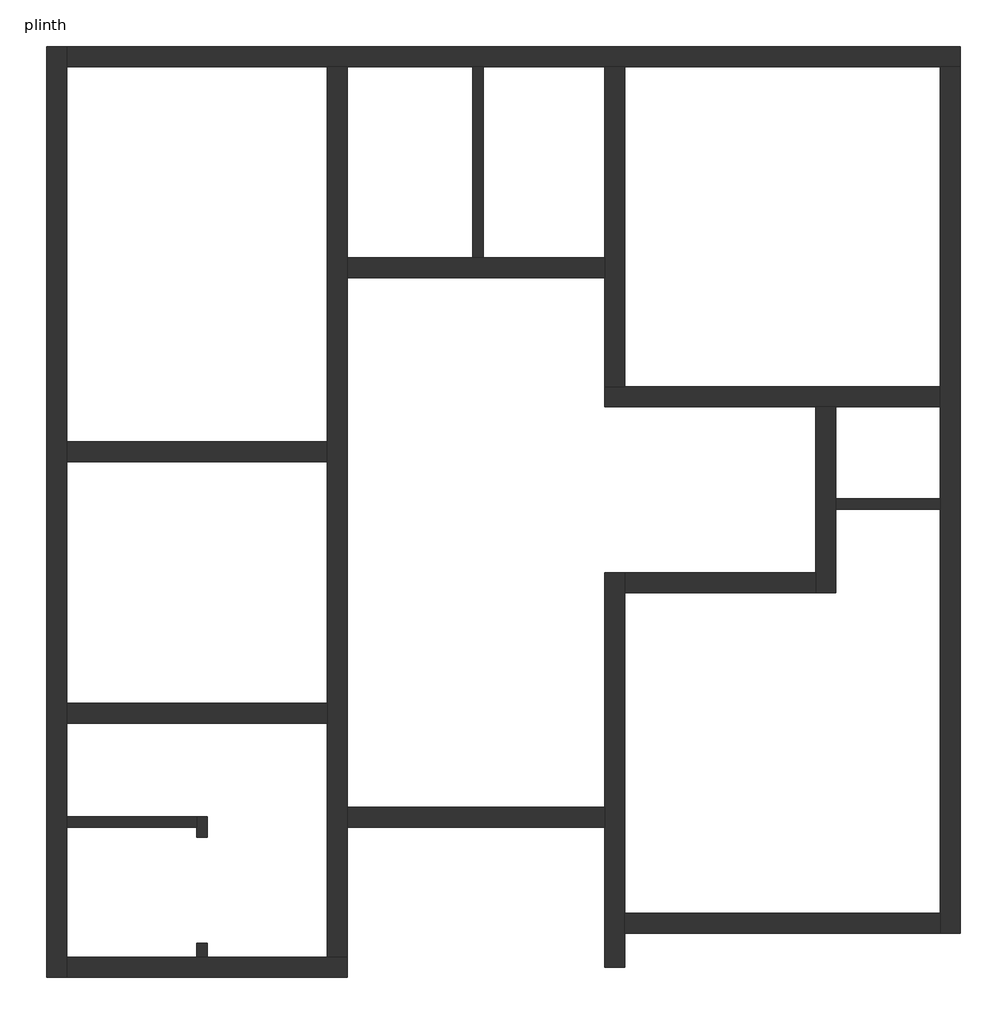
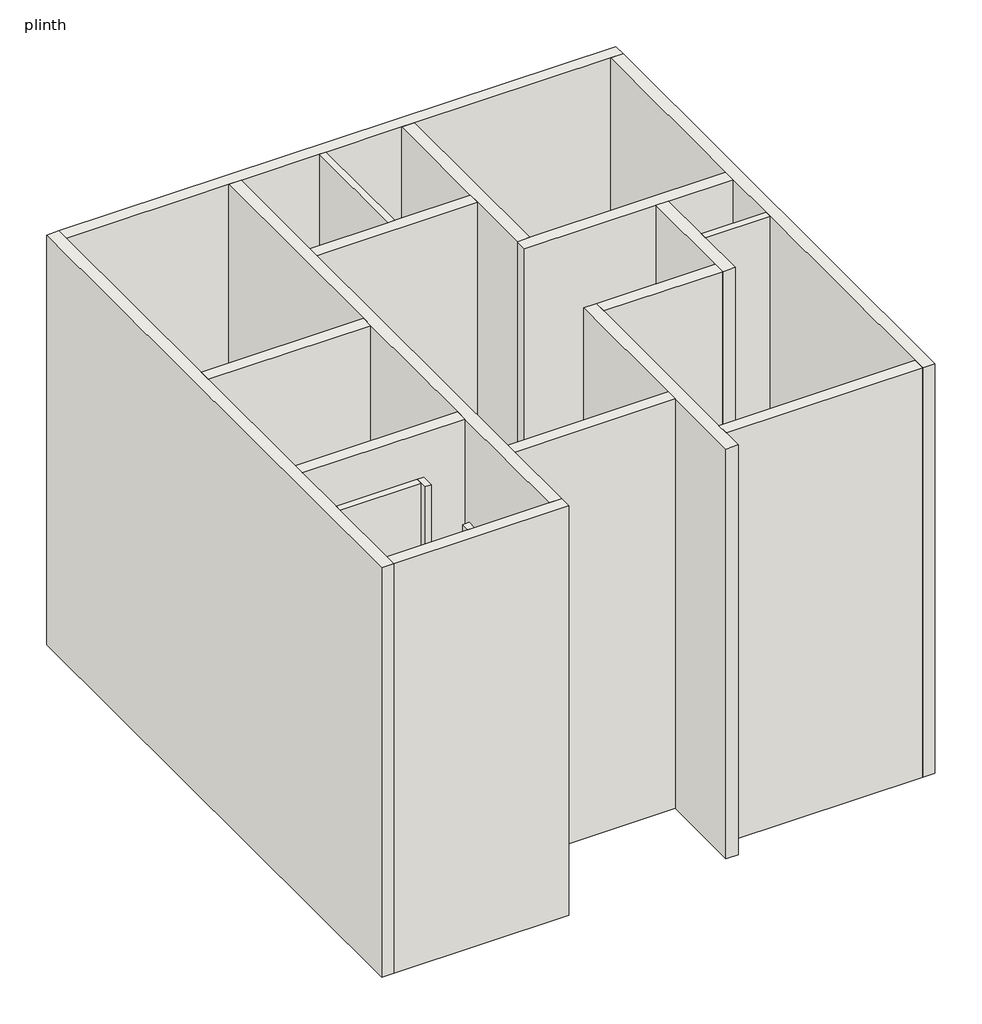
# One storey: 20 walls.
"""IFC4 building model written with IfcOpenShell, lengths in millimetres."""

from ifc_helpers import new_model, si_unit, frame, origin, place, context, project, spatial, polyline, outline, extrude, faceted_brep, element, save

model = new_model("IFC4")

# Units and contexts
model_context = context("Model", 3, world=origin())
ifc_project = project(units=[si_unit("LENGTHUNIT", "METRE", prefix="MILLI")], contexts=[model_context])

# Site, building, storey
site = spatial("IfcSite", under=ifc_project)
building = spatial("IfcBuilding", under=site)
storey = spatial("IfcBuildingStorey", under=building, Name="plinth", Elevation=450.0)

# Walls
placement = place(None, origin())
element("IfcWall", 1, ObjectType="11", at=placement, inside=storey, context=model_context, shape_type="SweptSolid", body=[
    extrude(outline(polyline([(-59261.991131, 24848.2615718), (-59261.991131, 22648.2615718), (-59381.991131, 22648.2615718), (-59381.991131, 24848.2615718), (-59261.991131, 24848.2615718)])), frame((0.0, 0.0, 450.0), z_axis=(0.0, 0.0, 1.0), x_axis=(1.0, 0.0, 0.0)), (0.0, 0.0, 1.0), 8000.0),
])
element("IfcWall", 2, ObjectType="111", at=placement, inside=storey, context=model_context, shape_type="SweptSolid", body=[
    extrude(outline(polyline([(-54001.991131, 19748.2615718), (-55201.991131, 19748.2615718), (-55201.991131, 19868.2615718), (-54001.991131, 19868.2615718), (-54001.991131, 19748.2615718)])), frame((0.0, 0.0, 450.0), z_axis=(0.0, 0.0, 1.0), x_axis=(1.0, 0.0, 0.0)), (0.0, 0.0, 1.0), 8000.0),
])
element("IfcWall", 3, ObjectType="111", at=placement, inside=storey, context=model_context, shape_type="Brep", body=[
    faceted_brep([(-62561.991131, 16208.2615718, 450.0), (-62561.991131, 16088.2615718, 450.0), (-62561.991131, 15973.2615718, 450.0), (-62561.991131, 15973.2615718, 8450.0), (-62561.991131, 16088.2615718, 8450.0), (-62561.991131, 16208.2615718, 8450.0), (-62441.991131, 16208.2615718, 450.0), (-62441.991131, 16208.2615718, 8450.0), (-62441.991131, 15973.2615718, 8450.0), (-62441.991131, 15973.2615718, 450.0)], [[[0, 1, 2, 3, 4, 5]], [[6, 7, 8, 9]], [[2, 1, 0, 6, 9]], [[3, 2, 9, 8]], [[5, 4, 3, 8, 7]], [[0, 5, 7, 6]]]),
])
element("IfcWall", 4, ObjectType="111", at=placement, inside=storey, context=model_context, shape_type="SweptSolid", body=[
    extrude(outline(polyline([(-62441.991131, 14753.2615718), (-62441.991131, 14588.2615718), (-62561.991131, 14588.2615718), (-62561.991131, 14753.2615718), (-62441.991131, 14753.2615718)])), frame((0.0, 0.0, 450.0), z_axis=(0.0, 0.0, 1.0), x_axis=(1.0, 0.0, 0.0)), (0.0, 0.0, 1.0), 8000.0),
])
element("IfcWall", 5, ObjectType="111", at=placement, inside=storey, context=model_context, shape_type="SweptSolid", body=[
    extrude(outline(polyline([(-64061.991131, 16208.2615718), (-62561.991131, 16208.2615718), (-62561.991131, 16088.2615718), (-64061.991131, 16088.2615718), (-64061.991131, 16208.2615718)])), frame((0.0, 0.0, 450.0), z_axis=(0.0, 0.0, 1.0), x_axis=(1.0, 0.0, 0.0)), (0.0, 0.0, 1.0), 8000.0),
])
element("IfcWall", 6, ObjectType="Generic - 200mm", at=placement, inside=storey, context=model_context, shape_type="Brep", body=[
    faceted_brep([(-64291.991131, 25078.2615718, 450.0), (-64291.991131, 14358.2615718, 450.0), (-64291.991131, 14358.2615718, 8450.0), (-64291.991131, 25078.2615718, 8450.0), (-64061.991131, 25078.2615718, 450.0), (-64061.991131, 25078.2615718, 8450.0), (-64061.991131, 24848.2615718, 8450.0), (-64061.991131, 20528.2615718, 8450.0), (-64061.991131, 20298.2615718, 8450.0), (-64061.991131, 17518.2615718, 8450.0), (-64061.991131, 17288.2615718, 8450.0), (-64061.991131, 16208.2615718, 8450.0), (-64061.991131, 16088.2615718, 8450.0), (-64061.991131, 14588.2615718, 8450.0), (-64061.991131, 14358.2615718, 8450.0), (-64061.991131, 14358.2615718, 450.0), (-64061.991131, 14588.2615718, 450.0), (-64061.991131, 16088.2615718, 450.0), (-64061.991131, 16208.2615718, 450.0), (-64061.991131, 17288.2615718, 450.0), (-64061.991131, 17518.2615718, 450.0), (-64061.991131, 20298.2615718, 450.0), (-64061.991131, 20528.2615718, 450.0), (-64061.991131, 24848.2615718, 450.0)], [[[0, 1, 2, 3]], [[4, 5, 6, 7, 8, 9, 10, 11, 12, 13, 14, 15, 16, 17, 18, 19, 20, 21, 22, 23]], [[1, 0, 4, 23, 22, 21, 20, 19, 18, 17, 16, 15]], [[3, 2, 14, 13, 12, 11, 10, 9, 8, 7, 6, 5]], [[2, 1, 15, 14]], [[0, 3, 5, 4]]]),
])
element("IfcWall", 7, ObjectType="Generic - 200mm", at=placement, inside=storey, context=model_context, shape_type="Brep", body=[
    faceted_brep([(-64061.991131, 14358.2615718, 450.0), (-60831.991131, 14358.2615718, 450.0), (-60831.991131, 14358.2615718, 8450.0), (-64061.991131, 14358.2615718, 8450.0), (-64061.991131, 14588.2615718, 450.0), (-64061.991131, 14588.2615718, 8450.0), (-62561.991131, 14588.2615718, 8450.0), (-62441.991131, 14588.2615718, 8450.0), (-61061.991131, 14588.2615718, 8450.0), (-60831.991131, 14588.2615718, 8450.0), (-60831.991131, 14588.2615718, 450.0), (-61061.991131, 14588.2615718, 450.0), (-62441.991131, 14588.2615718, 450.0), (-62561.991131, 14588.2615718, 450.0)], [[[0, 1, 2, 3]], [[4, 5, 6, 7, 8, 9, 10, 11, 12, 13]], [[1, 0, 4, 13, 12, 11, 10]], [[3, 2, 9, 8, 7, 6, 5]], [[0, 3, 5, 4]], [[2, 1, 10, 9]]]),
])
element("IfcWall", 8, ObjectType="Generic - 200mm", at=placement, inside=storey, context=model_context, shape_type="Brep", body=[
    faceted_brep([(-60831.991131, 14588.2615718, 450.0), (-60831.991131, 16088.2615718, 450.0), (-60831.991131, 16318.2615718, 450.0), (-60831.991131, 22418.2615718, 450.0), (-60831.991131, 22648.2615718, 450.0), (-60831.991131, 24848.2615718, 450.0), (-60831.991131, 24848.2615718, 8450.0), (-60831.991131, 22648.2615718, 8450.0), (-60831.991131, 22418.2615718, 8450.0), (-60831.991131, 16318.2615718, 8450.0), (-60831.991131, 16088.2615718, 8450.0), (-60831.991131, 14588.2615718, 8450.0), (-61061.991131, 14588.2615718, 450.0), (-61061.991131, 14588.2615718, 8450.0), (-61061.991131, 17288.2615718, 8450.0), (-61061.991131, 17518.2615718, 8450.0), (-61061.991131, 20298.2615718, 8450.0), (-61061.991131, 20528.2615718, 8450.0), (-61061.991131, 24848.2615718, 8450.0), (-61061.991131, 24848.2615718, 450.0), (-61061.991131, 20528.2615718, 450.0), (-61061.991131, 20298.2615718, 450.0), (-61061.991131, 17518.2615718, 450.0), (-61061.991131, 17288.2615718, 450.0)], [[[0, 1, 2, 3, 4, 5, 6, 7, 8, 9, 10, 11]], [[12, 13, 14, 15, 16, 17, 18, 19, 20, 21, 22, 23]], [[5, 4, 3, 2, 1, 0, 12, 23, 22, 21, 20, 19]], [[11, 10, 9, 8, 7, 6, 18, 17, 16, 15, 14, 13]], [[6, 5, 19, 18]], [[0, 11, 13, 12]]]),
])
element("IfcWall", 9, ObjectType="Generic - 200mm", at=placement, inside=storey, context=model_context, shape_type="Brep", body=[
    faceted_brep([(-53771.991131, 25078.2615718, 450.0), (-64061.991131, 25078.2615718, 450.0), (-64061.991131, 25078.2615718, 8450.0), (-53771.991131, 25078.2615718, 8450.0), (-53771.991131, 24848.2615718, 450.0), (-53771.991131, 24848.2615718, 8450.0), (-54001.991131, 24848.2615718, 8450.0), (-57631.991131, 24848.2615718, 8450.0), (-57861.991131, 24848.2615718, 8450.0), (-59261.991131, 24848.2615718, 8450.0), (-59381.991131, 24848.2615718, 8450.0), (-60831.991131, 24848.2615718, 8450.0), (-61061.991131, 24848.2615718, 8450.0), (-64061.991131, 24848.2615718, 8450.0), (-64061.991131, 24848.2615718, 450.0), (-61061.991131, 24848.2615718, 450.0), (-60831.991131, 24848.2615718, 450.0), (-59381.991131, 24848.2615718, 450.0), (-59261.991131, 24848.2615718, 450.0), (-57861.991131, 24848.2615718, 450.0), (-57631.991131, 24848.2615718, 450.0), (-54001.991131, 24848.2615718, 450.0)], [[[0, 1, 2, 3]], [[4, 5, 6, 7, 8, 9, 10, 11, 12, 13, 14, 15, 16, 17, 18, 19, 20, 21]], [[1, 0, 4, 21, 20, 19, 18, 17, 16, 15, 14]], [[3, 2, 13, 12, 11, 10, 9, 8, 7, 6, 5]], [[2, 1, 14, 13]], [[0, 3, 5, 4]]]),
])
element("IfcWall", 10, ObjectType="Generic - 200mm", at=placement, inside=storey, context=model_context, shape_type="Brep", body=[
    faceted_brep([(-54001.991131, 24848.2615718, 450.0), (-54001.991131, 21158.2615718, 450.0), (-54001.991131, 20928.2615718, 450.0), (-54001.991131, 19868.2615718, 450.0), (-54001.991131, 19748.2615718, 450.0), (-54001.991131, 15098.2615718, 450.0), (-54001.991131, 14868.2615718, 450.0), (-54001.991131, 14868.2615718, 8450.0), (-54001.991131, 15098.2615718, 8450.0), (-54001.991131, 19748.2615718, 8450.0), (-54001.991131, 19868.2615718, 8450.0), (-54001.991131, 20928.2615718, 8450.0), (-54001.991131, 21158.2615718, 8450.0), (-54001.991131, 24848.2615718, 8450.0), (-53771.991131, 24848.2615718, 450.0), (-53771.991131, 24848.2615718, 8450.0), (-53771.991131, 14868.2615718, 8450.0), (-53771.991131, 14868.2615718, 450.0)], [[[0, 1, 2, 3, 4, 5, 6, 7, 8, 9, 10, 11, 12, 13]], [[14, 15, 16, 17]], [[6, 5, 4, 3, 2, 1, 0, 14, 17]], [[13, 12, 11, 10, 9, 8, 7, 16, 15]], [[0, 13, 15, 14]], [[7, 6, 17, 16]]]),
])
element("IfcWall", 11, ObjectType="Generic - 200mm", at=placement, inside=storey, context=model_context, shape_type="Brep", body=[
    faceted_brep([(-54001.991131, 21158.2615718, 450.0), (-57631.991131, 21158.2615718, 450.0), (-57861.991131, 21158.2615718, 450.0), (-57861.991131, 21158.2615718, 8450.0), (-57631.991131, 21158.2615718, 8450.0), (-54001.991131, 21158.2615718, 8450.0), (-54001.991131, 20928.2615718, 450.0), (-54001.991131, 20928.2615718, 8450.0), (-55201.991131, 20928.2615718, 8450.0), (-55431.991131, 20928.2615718, 8450.0), (-57861.991131, 20928.2615718, 8450.0), (-57861.991131, 20928.2615718, 450.0), (-55431.991131, 20928.2615718, 450.0), (-55201.991131, 20928.2615718, 450.0)], [[[0, 1, 2, 3, 4, 5]], [[6, 7, 8, 9, 10, 11, 12, 13]], [[2, 1, 0, 6, 13, 12, 11]], [[5, 4, 3, 10, 9, 8, 7]], [[0, 5, 7, 6]], [[3, 2, 11, 10]]]),
])
element("IfcWall", 12, ObjectType="Generic - 200mm", at=placement, inside=storey, context=model_context, shape_type="SweptSolid", body=[
    extrude(outline(polyline([(-57631.991131, 15098.2615718), (-54001.991131, 15098.2615718), (-54001.991131, 14868.2615718), (-57631.991131, 14868.2615718), (-57631.991131, 15098.2615718)])), frame((0.0, 0.0, 450.0), z_axis=(0.0, 0.0, 1.0), x_axis=(1.0, 0.0, 0.0)), (0.0, 0.0, 1.0), 8000.0),
])
element("IfcWall", 13, ObjectType="Generic - 200mm", at=placement, inside=storey, context=model_context, shape_type="SweptSolid", body=[
    extrude(outline(polyline([(-57861.991131, 16088.2615718), (-60831.991131, 16088.2615718), (-60831.991131, 16318.2615718), (-57861.991131, 16318.2615718), (-57861.991131, 16088.2615718)])), frame((0.0, 0.0, 450.0), z_axis=(0.0, 0.0, 1.0), x_axis=(1.0, 0.0, 0.0)), (0.0, 0.0, 1.0), 8000.0),
])
element("IfcWall", 14, ObjectType="Generic - 200mm", at=placement, inside=storey, context=model_context, shape_type="SweptSolid", body=[
    extrude(outline(polyline([(-64061.991131, 17518.2615718), (-61061.991131, 17518.2615718), (-61061.991131, 17288.2615718), (-64061.991131, 17288.2615718), (-64061.991131, 17518.2615718)])), frame((0.0, 0.0, 450.0), z_axis=(0.0, 0.0, 1.0), x_axis=(1.0, 0.0, 0.0)), (0.0, 0.0, 1.0), 8000.0),
])
element("IfcWall", 15, ObjectType="Generic - 200mm", at=placement, inside=storey, context=model_context, shape_type="SweptSolid", body=[
    extrude(outline(polyline([(-64061.991131, 20528.2615718), (-61061.991131, 20528.2615718), (-61061.991131, 20298.2615718), (-64061.991131, 20298.2615718), (-64061.991131, 20528.2615718)])), frame((0.0, 0.0, 450.0), z_axis=(0.0, 0.0, 1.0), x_axis=(1.0, 0.0, 0.0)), (0.0, 0.0, 1.0), 8000.0),
])
element("IfcWall", 16, ObjectType="Generic - 200mm", at=placement, inside=storey, context=model_context, shape_type="Brep", body=[
    faceted_brep([(-57861.991131, 22648.2615718, 450.0), (-59261.991131, 22648.2615718, 450.0), (-59381.991131, 22648.2615718, 450.0), (-60831.991131, 22648.2615718, 450.0), (-60831.991131, 22648.2615718, 8450.0), (-59381.991131, 22648.2615718, 8450.0), (-59261.991131, 22648.2615718, 8450.0), (-57861.991131, 22648.2615718, 8450.0), (-57861.991131, 22418.2615718, 450.0), (-57861.991131, 22418.2615718, 8450.0), (-60831.991131, 22418.2615718, 8450.0), (-60831.991131, 22418.2615718, 450.0)], [[[0, 1, 2, 3, 4, 5, 6, 7]], [[8, 9, 10, 11]], [[3, 2, 1, 0, 8, 11]], [[7, 6, 5, 4, 10, 9]], [[4, 3, 11, 10]], [[0, 7, 9, 8]]]),
])
element("IfcWall", 17, ObjectType="Generic - 200mm", at=placement, inside=storey, context=model_context, shape_type="Brep", body=[
    faceted_brep([(-57861.991131, 19018.2615718, 450.0), (-57861.991131, 16318.2615718, 450.0), (-57861.991131, 16088.2615718, 450.0), (-57861.991131, 14473.2615718, 450.0), (-57861.991131, 14473.2615718, 8450.0), (-57861.991131, 16088.2615718, 8450.0), (-57861.991131, 16318.2615718, 8450.0), (-57861.991131, 19018.2615718, 8450.0), (-57631.991131, 19018.2615718, 450.0), (-57631.991131, 19018.2615718, 8450.0), (-57631.991131, 18788.2615718, 8450.0), (-57631.991131, 15098.2615718, 8450.0), (-57631.991131, 14868.2615718, 8450.0), (-57631.991131, 14473.2615718, 8450.0), (-57631.991131, 14473.2615718, 450.0), (-57631.991131, 14868.2615718, 450.0), (-57631.991131, 15098.2615718, 450.0), (-57631.991131, 18788.2615718, 450.0)], [[[0, 1, 2, 3, 4, 5, 6, 7]], [[8, 9, 10, 11, 12, 13, 14, 15, 16, 17]], [[3, 2, 1, 0, 8, 17, 16, 15, 14]], [[4, 3, 14, 13]], [[7, 6, 5, 4, 13, 12, 11, 10, 9]], [[0, 7, 9, 8]]]),
])
element("IfcWall", 18, ObjectType="Generic - 200mm", at=placement, inside=storey, context=model_context, shape_type="Brep", body=[
    faceted_brep([(-57631.991131, 21158.2615718, 450.0), (-57631.991131, 24848.2615718, 450.0), (-57631.991131, 24848.2615718, 8450.0), (-57631.991131, 21158.2615718, 8450.0), (-57861.991131, 21158.2615718, 450.0), (-57861.991131, 21158.2615718, 8450.0), (-57861.991131, 22418.2615718, 8450.0), (-57861.991131, 22648.2615718, 8450.0), (-57861.991131, 24848.2615718, 8450.0), (-57861.991131, 24848.2615718, 450.0), (-57861.991131, 22648.2615718, 450.0), (-57861.991131, 22418.2615718, 450.0)], [[[0, 1, 2, 3]], [[4, 5, 6, 7, 8, 9, 10, 11]], [[1, 0, 4, 11, 10, 9]], [[3, 2, 8, 7, 6, 5]], [[0, 3, 5, 4]], [[2, 1, 9, 8]]]),
])
element("IfcWall", 19, ObjectType="Generic - 200mm", at=placement, inside=storey, context=model_context, shape_type="Brep", body=[
    faceted_brep([(-55201.991131, 18788.2615718, 450.0), (-55201.991131, 19748.2615718, 450.0), (-55201.991131, 19868.2615718, 450.0), (-55201.991131, 20928.2615718, 450.0), (-55201.991131, 20928.2615718, 8450.0), (-55201.991131, 19868.2615718, 8450.0), (-55201.991131, 19748.2615718, 8450.0), (-55201.991131, 18788.2615718, 8450.0), (-55431.991131, 18788.2615718, 450.0), (-55431.991131, 18788.2615718, 8450.0), (-55431.991131, 19018.2615718, 8450.0), (-55431.991131, 20928.2615718, 8450.0), (-55431.991131, 20928.2615718, 450.0), (-55431.991131, 19018.2615718, 450.0)], [[[0, 1, 2, 3, 4, 5, 6, 7]], [[8, 9, 10, 11, 12, 13]], [[3, 2, 1, 0, 8, 13, 12]], [[7, 6, 5, 4, 11, 10, 9]], [[4, 3, 12, 11]], [[0, 7, 9, 8]]]),
])
element("IfcWall", 20, ObjectType="Generic - 200mm", at=placement, inside=storey, context=model_context, shape_type="SweptSolid", body=[
    extrude(outline(polyline([(-55431.991131, 18788.2615718), (-57631.991131, 18788.2615718), (-57631.991131, 19018.2615718), (-55431.991131, 19018.2615718), (-55431.991131, 18788.2615718)])), frame((0.0, 0.0, 450.0), z_axis=(0.0, 0.0, 1.0), x_axis=(1.0, 0.0, 0.0)), (0.0, 0.0, 1.0), 8000.0),
])

save(model, "model.ifc")

# Revit data of these elements
# Project information
#   Project Issue Date = "Issue Date"
#   Project Status = "Project Status"
#   Client Name = "Owner"
#   Project Address = "Enter address here"
#   Project Name = "Project Name"
#   Project Number = "0001"
# Type "11"
#   Layers, outside or top first: 1 cm no material (function 1); 10 cm no material (function 1); 1 cm no material (function 1)
# Type "111"
#   Layers, outside or top first: 1 cm no material (function 1); 10 cm no material (function 1); 1 cm no material (function 1)
# Type "Generic - 200mm"
#   Layers, outside or top first: 1.5 cm no material (function 1); 20 cm no material (function 1); 1.5 cm no material (function 1)
# Element 1 (IfcWall, "11")
#   Top Offset = 0 cm
#   Base Offset = 0 cm
#   Unconnected Height = 800 cm
#   wall height = 800 cm
#   Phase Created = New Construction
#   Base Constraint = plinth
#   Materials on its faces: "Default Wall"
# Elements 2, 3, 4, 5 (IfcWall, "111")
#   Top Offset = 0 cm
#   Base Offset = 0 cm
#   Unconnected Height = 800 cm
#   wall height = 800 cm
#   Phase Created = New Construction
#   Base Constraint = plinth
#   Materials on its faces: "Default Wall"
# Elements 6, 7, 8, 9, 10, 11, 12, 13, 14, 15, 16, 17, 18, 19, 20 (IfcWall, "Generic - 200mm")
#   Top Offset = 0 cm
#   Base Offset = 0 cm
#   Unconnected Height = 800 cm
#   wall height = 800 cm
#   Phase Created = New Construction
#   Base Constraint = plinth
#   Materials on its faces: "Default Wall"
# Materials
#   "Default Wall": class "Miscellaneous", colour RGB 128 128 128, transparency 0, Cost = 0
